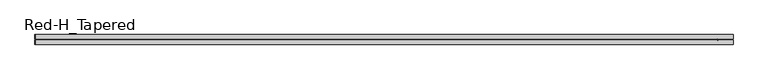
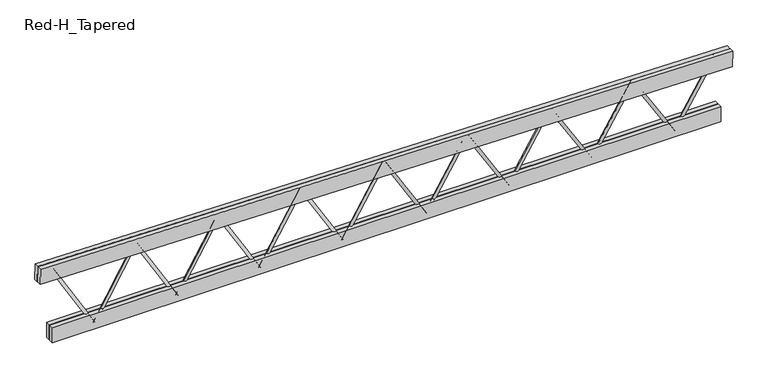
"""IFC4 building model written with IfcOpenShell, lengths in millimetres: beam geometry, Construction_Frames_RedBuilt_Openweb_Red-H_Tapered : Red-H_Tapered."""

from ifc_helpers import new_model, si_unit, point, frame, origin, origin_2d, place, context, project, spatial, polyline, circle_curve, trimmed, segment, composite_curve, outline, extrude, source, transform, mapped, element, save


def red_h_tapered_e83ac75d(model_context):
    return source(origin(), model_context, "Body", "SweptSolid", [
        extrude(outline(composite_curve([segment(trimmed(circle_curve(origin_2d(), 12.7), [point((0.0, 12.7))], [point((0.0, -12.7))], False, "CARTESIAN"), True, "CONTINUOUS"), segment(trimmed(circle_curve(origin_2d(), 12.7), [point((0.0, -12.7))], [point((0.0, 12.7))], False, "CARTESIAN"), True, "CONTINUOUS")], self_intersect=False)), frame((2514.6356775, 0.0, -367.0101562), z_axis=(0.5238075847033281, 0.0, 0.8518366123895273), x_axis=(0.0, -1.0, 0.0)), (0.0, 0.0, 1.0), 685.812269),
        extrude(outline(composite_curve([segment(trimmed(circle_curve(origin_2d(), 12.7), [point((0.0, -12.7))], [point((0.0, 12.6999999))], False, "CARTESIAN"), True, "CONTINUOUS"), segment(trimmed(circle_curve(origin_2d(), 12.7), [point((0.0, 12.6999999))], [point((0.0, -12.7))], False, "CARTESIAN"), True, "CONTINUOUS")], self_intersect=False)), frame((2514.6356775, 0.0, -367.0101562), z_axis=(-0.5212365661564261, 0.0, 0.8534122345627918), x_axis=(0.0, -1.0, 0.0)), (0.0, 0.0, 1.0), 689.1950633),
        extrude(outline(composite_curve([segment(trimmed(circle_curve(origin_2d(), 12.7), [point((0.0, 12.7))], [point((0.0, -12.6999999))], False, "CARTESIAN"), True, "CONTINUOUS"), segment(trimmed(circle_curve(origin_2d(), 12.7), [point((0.0, -12.6999999))], [point((0.0, 12.7))], False, "CARTESIAN"), True, "CONTINUOUS")], self_intersect=False)), frame((1796.168341, 0.0, -367.0101562), z_axis=(0.5212365661564254, 0.0, 0.8534122345627924), x_axis=(0.0, -1.0, 0.0)), (0.0, 0.0, 1.0), 689.1950633),
        extrude(outline(composite_curve([segment(trimmed(circle_curve(origin_2d(), 12.7), [point((0.0, -12.7))], [point((0.0, 12.7000001))], False, "CARTESIAN"), True, "CONTINUOUS"), segment(trimmed(circle_curve(origin_2d(), 12.7), [point((0.0, 12.7000001))], [point((0.0, -12.7))], False, "CARTESIAN"), True, "CONTINUOUS")], self_intersect=False)), frame((1796.168341, 0.0, -367.0101562), z_axis=(-0.51868601576627, 0.0, 0.8549648045671311), x_axis=(0.0, -1.0, 0.0)), (0.0, 0.0, 1.0), 692.584063),
        extrude(outline(composite_curve([segment(trimmed(circle_curve(origin_2d(), 12.7), [point((0.0, 12.7))], [point((0.0, -12.7))], False, "CARTESIAN"), True, "CONTINUOUS"), segment(trimmed(circle_curve(origin_2d(), 12.7), [point((0.0, -12.7))], [point((0.0, 12.7))], False, "CARTESIAN"), True, "CONTINUOUS")], self_intersect=False)), frame((1077.7010046, 0.0, -367.0101562), z_axis=(0.5186860157662689, 0.0, 0.8549648045671318), x_axis=(0.0, -1.0, 0.0)), (0.0, 0.0, 1.0), 692.584063),
        extrude(outline(composite_curve([segment(trimmed(circle_curve(origin_2d(), 12.7), [point((0.0, -12.7))], [point((0.0, 12.7))], False, "CARTESIAN"), True, "CONTINUOUS"), segment(trimmed(circle_curve(origin_2d(), 12.7), [point((0.0, 12.7))], [point((0.0, -12.7))], False, "CARTESIAN"), True, "CONTINUOUS")], self_intersect=False)), frame((1077.7010046, 0.0, -367.0101562), z_axis=(-0.5161557699811393, 0.0, 0.8564947291812001), x_axis=(0.0, -1.0, 0.0)), (0.0, 0.0, 1.0), 695.9791774),
        extrude(outline(composite_curve([segment(trimmed(circle_curve(origin_2d(), 12.7), [point((0.0, 12.7))], [point((0.0, -12.7))], False, "CARTESIAN"), True, "CONTINUOUS"), segment(trimmed(circle_curve(origin_2d(), 12.7), [point((0.0, -12.7))], [point((0.0, 12.7))], False, "CARTESIAN"), True, "CONTINUOUS")], self_intersect=False)), frame((359.2336682, 0.0, -367.0101562), z_axis=(0.5161557699811399, 0.0, 0.8564947291811997), x_axis=(0.0, -1.0, 0.0)), (0.0, 0.0, 1.0), 695.9791774),
        extrude(outline(composite_curve([segment(trimmed(circle_curve(origin_2d(), 12.7), [point((0.0, -12.7000001))], [point((0.0, 12.7))], False, "CARTESIAN"), True, "CONTINUOUS"), segment(trimmed(circle_curve(origin_2d(), 12.7), [point((0.0, 12.7))], [point((0.0, -12.7000001))], False, "CARTESIAN"), True, "CONTINUOUS")], self_intersect=False)), frame((359.2336682, 0.0, -367.0101562), z_axis=(-0.5136456648662128, 0.0, 0.8580024073183864), x_axis=(0.0, -1.0, 0.0)), (0.0, 0.0, 1.0), 699.3803176),
        extrude(outline(composite_curve([segment(trimmed(circle_curve(origin_2d(), 12.7), [point((0.0, -12.7))], [point((0.0, 12.7000001))], False, "CARTESIAN"), True, "CONTINUOUS"), segment(trimmed(circle_curve(origin_2d(), 12.7), [point((0.0, 12.7000001))], [point((0.0, -12.7))], False, "CARTESIAN"), True, "CONTINUOUS")], self_intersect=False)), frame((-359.2336682, 0.0, -367.0101562), z_axis=(0.5136456648661812, 0.0, 0.8580024073184053), x_axis=(0.0, -1.0, 0.0)), (0.0, 0.0, 1.0), 699.3803176),
        extrude(outline(composite_curve([segment(trimmed(circle_curve(origin_2d(), 12.7), [point((0.0, 12.7))], [point((0.0, -12.7))], False, "CARTESIAN"), True, "CONTINUOUS"), segment(trimmed(circle_curve(origin_2d(), 12.7), [point((0.0, -12.7))], [point((0.0, 12.7))], False, "CARTESIAN"), True, "CONTINUOUS")], self_intersect=False)), frame((-359.2336682, 0.0, -367.0101562), z_axis=(-0.5111555362037723, 0.0, 0.8594882301743486), x_axis=(0.0, -1.0, 0.0)), (0.0, 0.0, 1.0), 702.7873959),
        extrude(outline(composite_curve([segment(trimmed(circle_curve(origin_2d(), 12.7), [point((0.0, -12.7000001))], [point((0.0, 12.7))], False, "CARTESIAN"), True, "CONTINUOUS"), segment(trimmed(circle_curve(origin_2d(), 12.7), [point((0.0, 12.7))], [point((0.0, -12.7000001))], False, "CARTESIAN"), True, "CONTINUOUS")], self_intersect=False)), frame((-1077.7010046, 0.0, -367.0101562), z_axis=(0.5111555362037707, 0.0, 0.8594882301743495), x_axis=(0.0, -1.0, 0.0)), (0.0, 0.0, 1.0), 702.7873959),
        extrude(outline(composite_curve([segment(trimmed(circle_curve(origin_2d(), 12.7), [point((0.0, 12.7))], [point((0.0, -12.7))], False, "CARTESIAN"), True, "CONTINUOUS"), segment(trimmed(circle_curve(origin_2d(), 12.7), [point((0.0, -12.7))], [point((0.0, 12.7))], False, "CARTESIAN"), True, "CONTINUOUS")], self_intersect=False)), frame((-1077.7010046, 0.0, -367.0101562), z_axis=(-0.5086852195886448, 0.0, 0.8609525813725472), x_axis=(0.0, -1.0, 0.0)), (0.0, 0.0, 1.0), 706.2003266),
        extrude(outline(composite_curve([segment(trimmed(circle_curve(origin_2d(), 12.7), [point((0.0, -12.7))], [point((0.0, 12.6999999))], False, "CARTESIAN"), True, "CONTINUOUS"), segment(trimmed(circle_curve(origin_2d(), 12.7), [point((0.0, 12.6999999))], [point((0.0, -12.7))], False, "CARTESIAN"), True, "CONTINUOUS")], self_intersect=False)), frame((-1796.168341, 0.0, -367.0101562), z_axis=(0.5086852195886579, 0.0, 0.8609525813725394), x_axis=(0.0, -1.0, 0.0)), (0.0, 0.0, 1.0), 706.2003266),
        extrude(outline(composite_curve([segment(trimmed(circle_curve(origin_2d(), 12.7), [point((0.0, 12.6999999))], [point((0.0, -12.7000001))], False, "CARTESIAN"), True, "CONTINUOUS"), segment(trimmed(circle_curve(origin_2d(), 12.7), [point((0.0, -12.7000001))], [point((0.0, 12.6999999))], False, "CARTESIAN"), True, "CONTINUOUS")], self_intersect=False)), frame((-1796.168341, 0.0, -367.0101562), z_axis=(-0.5062345505185052, 0.0, 0.862395837108069), x_axis=(0.0, -1.0, 0.0)), (0.0, 0.0, 1.0), 709.6190251),
        extrude(outline(composite_curve([segment(trimmed(circle_curve(origin_2d(), 12.7), [point((0.0, -12.6999999))], [point((0.0, 12.7000001))], False, "CARTESIAN"), True, "CONTINUOUS"), segment(trimmed(circle_curve(origin_2d(), 12.7), [point((0.0, 12.7000001))], [point((0.0, -12.6999999))], False, "CARTESIAN"), True, "CONTINUOUS")], self_intersect=False)), frame((-2514.6356775, 0.0, -367.0101562), z_axis=(0.5062345505184935, 0.0, 0.8623958371080759), x_axis=(0.0, -1.0, 0.0)), (0.0, 0.0, 1.0), 709.6190251),
        extrude(outline(composite_curve([segment(trimmed(circle_curve(origin_2d(), 12.7), [point((0.0, 12.7))], [point((0.0, -12.7))], False, "CARTESIAN"), True, "CONTINUOUS"), segment(trimmed(circle_curve(origin_2d(), 12.7), [point((0.0, -12.7))], [point((0.0, 12.7))], False, "CARTESIAN"), True, "CONTINUOUS")], self_intersect=False)), frame((-2514.6356775, 0.0, -367.0101562), z_axis=(-0.5038033644797613, 0.0, 0.8638183662893912), x_axis=(0.0, -1.0, 0.0)), (0.0, 0.0, 1.0), 713.0434085),
        extrude(outline(polyline([(-2899.2693457, -41.275), (-2899.2693457, -3.175), (2899.2693457, -3.175), (2899.2693457, -41.275), (-2899.2693457, -41.275)])), frame((0.0, 0.0, -386.0601562), z_axis=(0.0, 0.0, 1.0), x_axis=(1.0, 0.0, 0.0)), (0.0, 0.0, 1.0), 139.7),
        extrude(outline(polyline([(-2899.2693457, 3.175), (-2899.2693457, 41.275), (2899.2693457, 41.275), (2899.2693457, 3.175), (-2899.2693457, 3.175)])), frame((0.0, 0.0, -386.0601562), z_axis=(0.0, 0.0, 1.0), x_axis=(1.0, 0.0, 0.0)), (0.0, 0.0, 1.0), 139.7),
        extrude(outline(polyline([(0.0, -38.1), (0.0, 0.0), (6002.5985939, 0.0), (6002.5985939, -38.1), (0.0, -38.1)])), frame((-3003.2339083, -3.175, 185.4598565), z_axis=(0.01692600269882894, 0.0, 0.9998567449553157), x_axis=(0.9998567449553157, 0.0, -0.01692600269882894)), (0.0, 0.0, 1.0), 139.7),
        extrude(outline(polyline([(0.0, -38.1), (0.0, 0.0), (6002.5985939, 0.0), (6002.5985939, -38.1), (0.0, -38.1)])), frame((-3003.2339083, 41.275, 185.4598565), z_axis=(0.01692600269882894, 0.0, 0.9998567449553157), x_axis=(0.9998567449553157, 0.0, -0.01692600269882894)), (0.0, 0.0, 1.0), 139.7),
    ])


if __name__ == "__main__":
    model = new_model("IFC4")
    model_context = context("Model", 3, world=origin())
    ifc_project = project(units=[si_unit("LENGTHUNIT", "METRE", prefix="MILLI")], contexts=[model_context])
    site = spatial("IfcSite", under=ifc_project)
    building = spatial("IfcBuilding", under=site)
    placement = place(None, origin())
    red_h_tapered_shape = red_h_tapered_e83ac75d(model_context)
    element("IfcBeam", 1, ObjectType="Construction_Frames_RedBuilt_Openweb_Red-H_Tapered : Red-H_Tapered", at=placement, inside=building, context=model_context, shape_type="MappedRepresentation", body=[
        mapped(red_h_tapered_shape, transform((0.0, 0.0, 0.0), x_axis=(1.0, 0.0, 0.0), y_axis=(0.0, 1.0, 0.0), z_axis=(0.0, 0.0, 1.0))),
    ])
    save(model, "model.ifc")

# Revit data of these elements
# Type "Construction_Frames_RedBuilt_Openweb_Red-H_Tapered : Red-H_Tapered"
#   Youtube clip = ""
#   Weight Net (Kg) = "0"
#   Webs = "Up to 2\" diameter tubular steel"
#   Uniformat II Description = ""
#   Uniformat II Code = ""
#   Uniclass 2015 Name = "Softwood trusses"
#   Uniclass 2015 Code = "Pr_20_85_90_81"
#   Uniclass 2.0 Description = "Structural Framing Systems"
#   Uniclass 2.0 Code = "SS-15-10-75"
#   Uniclass 1.4 Description = "Trusses"
#   Uniclass 1.4 Code = "L3523"
#   UNSPSC Code = "30103606"
#   Technical description = "http://www.redbuilt.com/reference/literature-and-other-resources"
#   Region South America = "None"
#   Region Oceania = "None"
#   Region North America = "US"
#   Region Middle East = "None"
#   Region Europe = "None"
#   Region Asia = "None"
#   Region Antarctica = "None"
#   Region Africa = "None"
#   QR code = "http://bimobject.com/redbuilt/product/redbuilt-0003"
#   Product url = "http://www.redbuilt.com/products/default.aspx?id=2"
#   Product group = "Wood Trusses"
#   Product family = "Construction"
#   Product data url = "https://bimobject.com/redbuilt/product/redbuilt-0003"
#   Product certification = ""
#   Product SKU = "redbuilt-0003"
#   Product Page URL = "http://www.redbuilt.com/commercial-systems/red-m-red-h-open-web-trusses"
#   Product Guid = "2c5793f2-6ffb-4665-b825-cf90c048e711"
#   Product Documentation Link = "http://www.redbuilt.com/documents/OW_Guide_2017_07_LowRes_wLinks.pdf"
#   OmniClass Description = "Wood Trusses"
#   OmniClass Code = "23-13 35 19 13 17"
#   NBS Reference Description = ""
#   NBS Reference Code = ""
#   Material secondary = "Steel"
#   Material main = "CHARRED WOOD"
#   Masterformat 2014 Description = "Metal-Web Wood Joists"
#   Masterformat 2014 Code = "06 17 36"
#   Manufacturer name = "RedBuilt"
#   Manufacturer country = "United States"
#   Installation instructions = "http://www.redbuilt.com/documents/Installation_Sheets_Open-Web.pdf"
#   IFC Classification = ""
#   EAN code = ""
#   Design country = "United States"
#   Product Information = "http://redbuilt.com/products/default.aspx?id=2"
#   Model = "Red-H-Tapered"
#   Manufacturer URL = "http://redbuilt.com/"
#   Manufacturer = "RedBuilt™"
#   Description = "Open Web Truss"
#   Date of publishing = "8/17/2010"
#   Contact us = "http://redbuilt.com/contact/"
#   Chords = "Double 1½\" x 5½\" MSR lumber"
#   COBIe Type Category = ""
#   Brand url = "http://www.redbuilt.com"
#   BIMobject main category code = "construction"
#   BIMobject main category = "Construction"
#   BIMobject category code = "construction-frames-trusses"
#   BIMobject category = "Frames & Trusses"
#   Web Radius = 0' - 0 1/2"
#   Web Layout Offset Start [instance default] = 0' - 5"
#   Web Layout Offset End [instance default] = 0' - 5"
#   Web Diameter = 0' - 1"
#   TotalLength [instance default] = 20' - 0"
#   Span Minimum = 4' - 0"
#   Span Maximum = 70' - 0"
#   Span Limit [instance default] = 20' - 0"
#   Nominal width = 0' - 0"
#   Nominal height = 0' - 0"
#   Inner Depth Top [instance default] = 0' - 2.76372"
#   Depth Start [instance default] = 6' - 0"
#   Top Chord Length [instance default] = 20' - 1.19701"
#   TC Extension Start Aux [instance default] = 0' - 0"
#   TC Extension End Aux [instance default] = 0' - 0"
#   T-B Chord Length Difference L [instance default] = 0' - 4"
#   T-B Chord Length Difference [instance default] = 0' - 4"
#   Height 2 [instance default] = 6' - 0"
#   Depth Minimum at Wall = 2' - 0"
#   Depth Maximum at Wall = 6' - 0"
#   Depth Lower End [instance default] = 2' - 0"
#   Depth Higher End [instance default] = 6' - 0"
#   Depth End [instance default] = 2' - 0"
#   Depth 2 [instance default] = 2' - 0"
#   Chord Width = 0' - 3 1/4"
#   Chord Thickness = 0' - 1 1/2"
#   Chord Depth = 0' - 5 1/2"
#   Offset Start [instance default] = 0' - 0"
#   TC Extension Start [instance default] = 0' - 0"
#   End Panel = 0' - 5"
#   Offset End [instance default] = 0' - 0"
#   TC Extension End [instance default] = 0' - 0"
#   Length [instance default] = 20' - 0"
#   Angle [instance default] = 5.71059°
#   Span Limit Warning [instance default] = no
#   Edition number = 1
#   Top Bearing Start [instance default] = yes
#   Top Bearing End [instance default] = yes
#   Bottom Bearing Start [instance default] = no
#   Bottom Bearing End [instance default] = no
#   8 Panels [instance default] = yes
#   16 Panels [instance default] = no
#   12 Panels [instance default] = no
#   Web Material = RedBuilt-Steel, Galvanized
#   Clip Material = RedBuilt-Steel, Galvanized
#   Chords Material = WOOD-OAKFIRE
#   URL = ""
#   Assembly Code = ""
# Element 1 (IfcBeam, "Construction_Frames_RedBuilt_Openweb_Red-H_Tapered : Red-H_Tapered")
#   TotalLength = 19' - 8.28892"
#   Span Limit = 19' - 8.28892"
#   Inner Depth Top = 0' - 2.75039"
#   Depth Start = 5' - 0"
#   Top Chord Length = 19' - 8.32278"
#   Height 2 = 5' - 0"
#   Depth Higher End = 5' - 0"
#   Depth 2 = 0' - 4"
#   Angle = 0.969835°
#   Materials on its faces: "RedBuilt-Steel, Galvanized", "WOOD-OAKFIRE"
# Materials
#   "RedBuilt-Steel, Galvanized": class "Metal", colour RGB 164 172 176, transparency 0, Manufacturer = "RedBuilt. LLC", Comments = "Openweb Metal Web", URL = "http://www.redbuilt.com/", Description = "Galvanized steel", Cost = 0
#   "WOOD-OAKFIRE": class "Wood", colour RGB 198 202 183, transparency 0, Description = "Generic wood", Cost = 0
